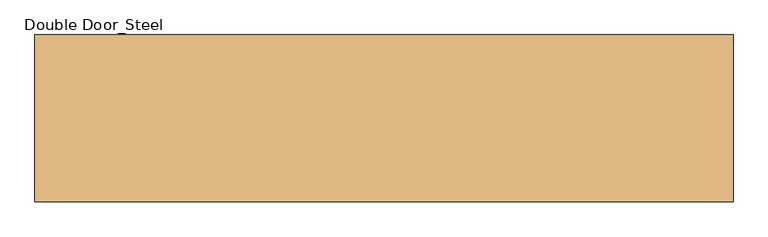
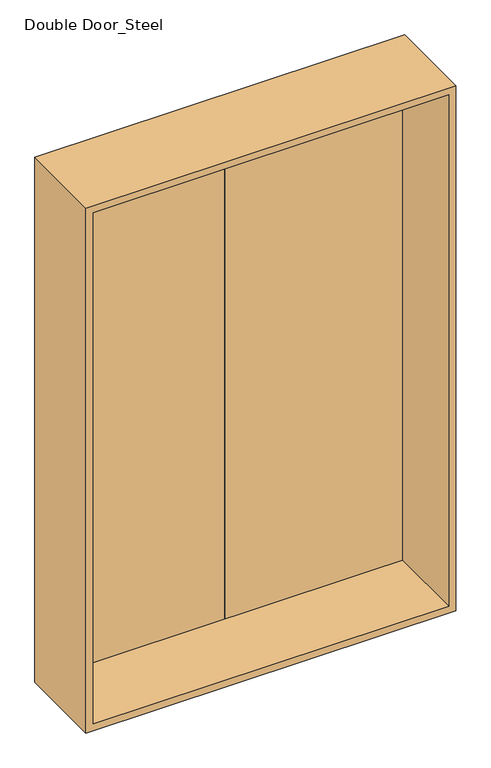
"""IFC4 building model written with IfcOpenShell, lengths in millimetres: door geometry, Double Door_Steel : H_DR_AMB_Double Door_Steel_W1800xH2700."""

from ifc_helpers import new_model, si_unit, frame, origin, place, context, project, spatial, polyline, outline, extrude, faceted_brep, source, transform, mapped, element, save


def double_door_steel_634f6038(model_context):
    return source(origin(), model_context, "Body", "SolidModel", [
        extrude(outline(polyline([(880.0, 175.0), (0.0, 175.0), (0.0, 215.0), (880.0, 215.0), (880.0, 175.0)])), frame((0.0, 0.0, 20.0), z_axis=(0.0, 0.0, 1.0), x_axis=(1.0, 0.0, 0.0)), (0.0, 0.0, 1.0), 2660.0),
        extrude(outline(polyline([(0.0, 175.0), (-880.0, 175.0), (-880.0, 215.0), (0.0, 215.0), (0.0, 175.0)])), frame((0.0, 0.0, 20.0), z_axis=(0.0, 0.0, 1.0), x_axis=(1.0, 0.0, 0.0)), (0.0, 0.0, 1.0), 2660.0),
        faceted_brep([(900.0, -215.0, 2700.0), (900.0, 215.0, 2700.0), (-900.0, 215.0, 2700.0), (-900.0, -215.0, 2700.0), (865.0, 175.0, 2665.0), (865.0, -215.0, 2665.0), (-865.0, -215.0, 2665.0), (-865.0, 175.0, 2665.0), (880.0, 215.0, 2680.0), (880.0, 175.0, 2680.0), (-880.0, 175.0, 2680.0), (-880.0, 215.0, 2680.0), (-900.0, 215.0, 0.0), (-900.0, -215.0, 0.0), (-865.0, -215.0, 35.0), (-865.0, 175.0, 35.0), (-880.0, 175.0, 20.0), (-880.0, 215.0, 20.0), (900.0, 215.0, 0.0), (880.0, 215.0, 20.0), (900.0, -215.0, 0.0), (865.0, -215.0, 35.0), (865.0, 175.0, 35.0), (880.0, 175.0, 20.0)], [[[0, 1, 2, 3]], [[4, 5, 6, 7]], [[8, 9, 10, 11]], [[3, 2, 12, 13]], [[7, 6, 14, 15]], [[11, 10, 16, 17]], [[18, 12, 2, 1], [8, 11, 17, 19]], [[13, 12, 18, 20]], [[0, 3, 13, 20], [21, 14, 6, 5]], [[15, 14, 21, 22]], [[23, 16, 10, 9], [4, 7, 15, 22]], [[17, 16, 23, 19]], [[20, 18, 1, 0]], [[22, 21, 5, 4]], [[19, 23, 9, 8]]]),
    ])


if __name__ == "__main__":
    model = new_model("IFC4")
    model_context = context("Model", 3, world=origin())
    ifc_project = project(units=[si_unit("LENGTHUNIT", "METRE", prefix="MILLI")], contexts=[model_context])
    site = spatial("IfcSite", under=ifc_project)
    building = spatial("IfcBuilding", under=site)
    placement = place(None, origin())
    double_door_steel_shape = double_door_steel_634f6038(model_context)
    element("IfcDoor", 1, ObjectType="Double Door_Steel : H_DR_AMB_Double Door_Steel_W1800xH2700", at=placement, inside=building, context=model_context, shape_type="MappedRepresentation", body=[
        mapped(double_door_steel_shape, transform((0.0, 0.0, 0.0), x_axis=(1.0, 0.0, 0.0), y_axis=(0.0, 1.0, 0.0), z_axis=(0.0, 0.0, 1.0))),
    ])
    save(model, "model.ifc")

# Revit data of these elements
# Type "Double Door_Steel : H_DR_AMB_Double Door_Steel_W1800xH2700"
#   Type Mark = "363"
#   프레임 = ""
#   철물 = ""
#   유리/마감 = ""
#   위치/개소 = ""
#   부호 = "1/SD"
#   문번호 = ""
#   문기호 = "SD"
#   Analytic Construction = "<None>"
#   Height = 2700.000 mm
#   Width = 1800.000 mm
#   Define Thermal Properties by = 1
#   문 틀 = none
#   문 = none
#   Function = (empty or 0)
#   Assembly Code = ""
#   Wall Closure = (empty or 0)
